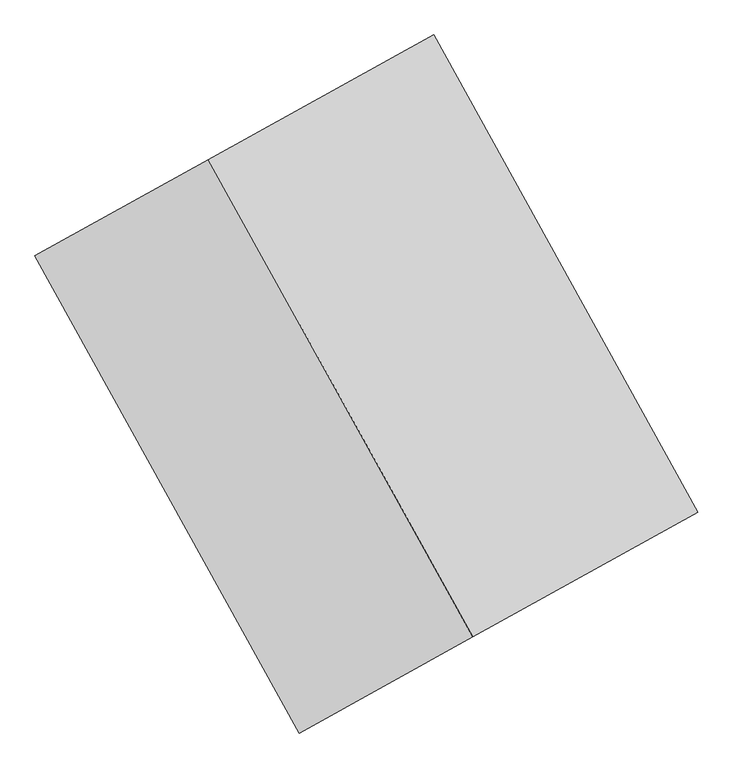
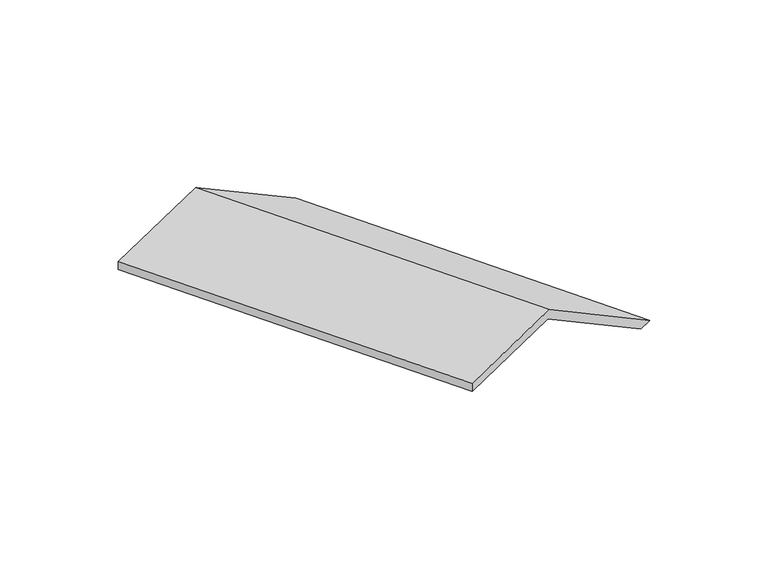
"""IFC4 building model written with IfcOpenShell, lengths in millimetres: beam geometry, KNA_SF_Talud 1 : KNA_SF_Talud 1."""

from ifc_helpers import new_model, si_unit, frame, origin, place, context, project, spatial, polyline, outline, extrude, source, transform, mapped, element, save


def beam_c0b1e3fd(model_context):
    return source(origin(), model_context, "Body", "SweptSolid", [
        extrude(outline(polyline([(7193.0875107, 0.0), (11032.9899199, -2559.9284026), (10866.5801552, -2809.543687), (7102.2550123, -300.0), (450.0011491, -300.0), (0.0, 0.0), (7193.0875107, 0.0)])), frame((132086.0138355, -50279.2958887, -1040.0), z_axis=(-0.48434294505380965, 0.8748782267130679, 0.0), x_axis=(-0.7279432579907724, -0.40299800662766855, 0.5546992156114027)), (0.0, 0.0, 1.0), 12696.9992738),
    ])


if __name__ == "__main__":
    model = new_model("IFC4")
    model_context = context("Model", 3, world=origin())
    ifc_project = project(units=[si_unit("LENGTHUNIT", "METRE", prefix="MILLI")], contexts=[model_context])
    site = spatial("IfcSite", under=ifc_project)
    building = spatial("IfcBuilding", under=site)
    placement = place(None, origin())
    beam_shape = beam_c0b1e3fd(model_context)
    element("IfcBeam", 1, ObjectType="KNA_SF_Talud 1 : KNA_SF_Talud 1", at=placement, inside=building, context=model_context, shape_type="MappedRepresentation", body=[
        mapped(beam_shape, transform((0.0, 0.0, 0.0), x_axis=(1.0, 0.0, 0.0), y_axis=(0.0, 1.0, 0.0), z_axis=(0.0, 0.0, 1.0))),
    ])
    save(model, "model.ifc")
